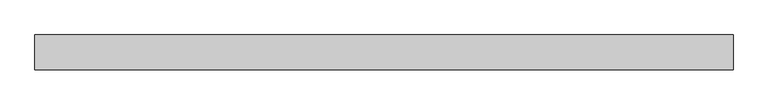
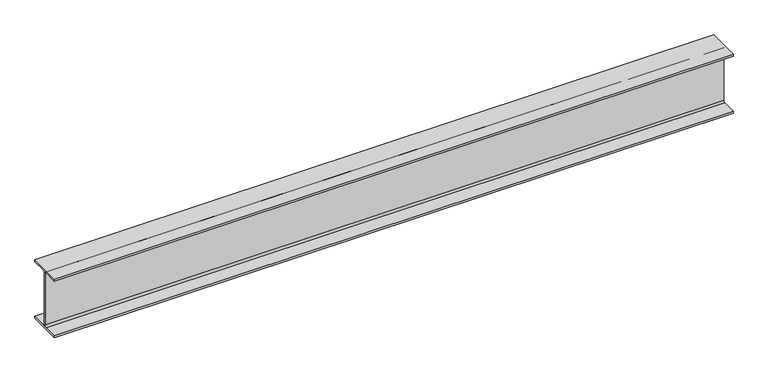
"""IFC4 building model written with IfcOpenShell, lengths in millimetres: beam geometry, Steel Beam_H-KSD3502 : H_SB_ASB_H-200x200x8x12."""

import ifcopenshell
import ifcopenshell.guid

model = None  # the IFC model being written
_history = None  # IfcOwnerHistory: only IFC2X3 demands one
_inside = {}  # id of a spatial element -> (the spatial element, [elements in it])
_under = {}  # id of a project, library or spatial element -> (it, [spatial elements below it])
_declared = {}  # id of a project -> (the project, [libraries it declares])
_typed = {}  # id of a type object -> (the type object, [elements of that type])
_made_of = {}  # id of a material, layer set ... -> (it, [elements and type objects made of it])


def new_model(schema):
    """Start an empty IFC model of exactly this schema.

    Asked for "IFC4X3", IfcOpenShell would pick the latest addendum, in which some entities
    have other attributes; the version numbers below select the first issue.
    IFC2X3 requires an IfcOwnerHistory on every rooted entity: one is made here for all.
    """
    global model, _history
    if schema == "IFC4X3":
        model = ifcopenshell.file(schema_version=(4, 3, 0, 0))
    else:
        model = ifcopenshell.file(schema=schema)
    _inside.clear()
    _under.clear()
    _declared.clear()
    _typed.clear()
    _made_of.clear()
    _history = None
    if model.schema == "IFC2X3":
        org = make("IfcOrganization", Name="unknown")
        user = make(
            "IfcPersonAndOrganization",
            ThePerson=make("IfcPerson", FamilyName="unknown"),
            TheOrganization=org,
        )
        app = make(
            "IfcApplication",
            ApplicationDeveloper=org,
            Version="unknown",
            ApplicationFullName="unknown",
            ApplicationIdentifier="unknown",
        )
        _history = make(
            "IfcOwnerHistory",
            OwningUser=user,
            OwningApplication=app,
            ChangeAction="ADDED",
            CreationDate=0,
        )
    return model


def make(cls, **values):
    """One entity of the class cls with the attributes given. An attribute that is None is left unset."""
    return model.create_entity(
        cls, **{name: value for name, value in values.items() if value is not None}
    )


def rooted(cls, **values):
    """An entity with a GlobalId (a new one), such as an element, a storey or a relation."""
    return make(cls, GlobalId=ifcopenshell.guid.new(), OwnerHistory=_history, **values)


def si_unit(unit_type, name, prefix=None):
    """IfcSIUnit, for example si_unit("LENGTHUNIT", "METRE", prefix="MILLI")."""
    return make("IfcSIUnit", UnitType=unit_type, Prefix=prefix, Name=name)


def assignment(units):
    """IfcUnitAssignment: the units of a project."""
    return None if units is None else make("IfcUnitAssignment", Units=units)


def point(xyz):
    """IfcCartesianPoint."""
    return None if xyz is None else make("IfcCartesianPoint", Coordinates=xyz)


def direction(xyz):
    """IfcDirection."""
    return None if xyz is None else make("IfcDirection", DirectionRatios=xyz)


def frame(location, z_axis=None, x_axis=None):
    """IfcAxis2Placement3D, a coordinate frame: its origin and axes. An axis left out is left unset."""
    return make(
        "IfcAxis2Placement3D",
        Location=point(location),
        Axis=direction(z_axis),
        RefDirection=direction(x_axis),
    )


def frame_2d(location, x_axis=None):
    """IfcAxis2Placement2D, a coordinate frame in the plane: its origin and x axis."""
    return make(
        "IfcAxis2Placement2D", Location=point(location), RefDirection=direction(x_axis)
    )


def origin():
    """The frame at (0, 0, 0) with its axes left unset."""
    return frame((0.0, 0.0, 0.0))


def place(relative_to, where):
    """IfcLocalPlacement: puts the frame where relative to a parent placement (None: the world)."""
    return make(
        "IfcLocalPlacement", PlacementRelTo=relative_to, RelativePlacement=where
    )


def context(
    kind, dimensions, precision=None, world=None, true_north=None, identifier=None
):
    """IfcGeometricRepresentationContext, for example the 3D "Model" context."""
    return make(
        "IfcGeometricRepresentationContext",
        ContextIdentifier=identifier,
        ContextType=kind,
        CoordinateSpaceDimension=dimensions,
        Precision=precision,
        WorldCoordinateSystem=world,
        TrueNorth=true_north,
    )


def project(units=None, contexts=None):
    """IfcProject with its units and contexts."""
    return rooted(
        "IfcProject",
        Name="project",
        RepresentationContexts=contexts,
        UnitsInContext=assignment(units),
    )


def spatial(cls, under=None, at=None, **own):
    """A site, building, storey or space (cls), placed at a placement, below another one or the project."""
    s = rooted(cls, ObjectPlacement=at, **own)
    if under is not None:
        _under.setdefault(under.id(), (under, []))[1].append(s)
    return s


def polyline(points):
    """IfcPolyline through the points."""
    return make("IfcPolyline", Points=[point(p) for p in points])


def circle_curve(where, radius):
    """IfcCircle in the frame where."""
    return make("IfcCircle", Position=where, Radius=radius)


def trimmed(basis, trim1, trim2, sense, master):
    """IfcTrimmedCurve: the piece of a basis curve between two trims."""
    return make(
        "IfcTrimmedCurve",
        BasisCurve=basis,
        Trim1=trim1,
        Trim2=trim2,
        SenseAgreement=sense,
        MasterRepresentation=master,
    )


def segment(curve, same_sense, transition):
    """IfcCompositeCurveSegment."""
    return make(
        "IfcCompositeCurveSegment",
        Transition=transition,
        SameSense=same_sense,
        ParentCurve=curve,
    )


def composite_curve(segments, self_intersect=None):
    """IfcCompositeCurve: segments joined end to end."""
    return make("IfcCompositeCurve", Segments=segments, SelfIntersect=self_intersect)


def outline(outer, holes=None, kind="AREA"):
    """IfcArbitraryClosedProfileDef: a profile drawn as a closed curve; with holes, ...WithVoids."""
    if holes is None:
        return make("IfcArbitraryClosedProfileDef", ProfileType=kind, OuterCurve=outer)
    return make(
        "IfcArbitraryProfileDefWithVoids",
        ProfileType=kind,
        OuterCurve=outer,
        InnerCurves=holes,
    )


def extrude(swept, where, along, depth):
    """IfcExtrudedAreaSolid: the profile swept, set in the frame where, extruded along a direction by depth."""
    return make(
        "IfcExtrudedAreaSolid",
        SweptArea=swept,
        Position=where,
        ExtrudedDirection=direction(along),
        Depth=depth,
    )


def shape(context_of_items, identifier, shape_type, items):
    """IfcShapeRepresentation: the items that make up one representation, for example the "Body"."""
    return make(
        "IfcShapeRepresentation",
        ContextOfItems=context_of_items,
        RepresentationIdentifier=identifier,
        RepresentationType=shape_type,
        Items=items,
    )


def source(mapping_origin, context_of_items, identifier, shape_type, items):
    """IfcRepresentationMap: a shape defined once, which mapped items show again and again."""
    return make(
        "IfcRepresentationMap",
        MappingOrigin=mapping_origin,
        MappedRepresentation=shape(context_of_items, identifier, shape_type, items),
    )


def transform(
    local_origin,
    x_axis=None,
    y_axis=None,
    z_axis=None,
    scale=None,
    scale2=None,
    scale3=None,
    uniform=True,
):
    """IfcCartesianTransformationOperator3D, or its non-uniform kind. x_axis, y_axis, z_axis: its Axis1, 2, 3."""
    if uniform:
        return make(
            "IfcCartesianTransformationOperator3D",
            Axis1=direction(x_axis),
            Axis2=direction(y_axis),
            LocalOrigin=point(local_origin),
            Scale=scale,
            Axis3=direction(z_axis),
        )
    return make(
        "IfcCartesianTransformationOperator3DnonUniform",
        Axis1=direction(x_axis),
        Axis2=direction(y_axis),
        LocalOrigin=point(local_origin),
        Scale=scale,
        Axis3=direction(z_axis),
        Scale2=scale2,
        Scale3=scale3,
    )


def mapped(mapping_source, mapping_target):
    """IfcMappedItem: shows the shape of a source again, moved by a transform."""
    return make(
        "IfcMappedItem", MappingSource=mapping_source, MappingTarget=mapping_target
    )


def made_of(thing, what):
    """Note that an element or type object is made of a material, layer set ...; save() writes the relation."""
    if what is not None:
        _made_of.setdefault(what.id(), (what, []))[1].append(thing)
    return thing


def element(
    cls,
    number,
    at=None,
    inside=None,
    cuts=None,
    type_object=None,
    material=None,
    context=None,
    identifier="Body",
    shape_type=None,
    held_by="IfcProductDefinitionShape",
    body=None,
    shapes=None,
    **own,
):
    """One element of the class cls, such as IfcWall. Its Tag is "e" and its number.

    at: its placement. inside: the storey or other place that contains it. cuts: it is an
    opening in that element (IfcRelVoidsElement). A single representation is given by context,
    identifier, shape_type and body (its items); several are given by shapes. held_by: the class
    of the entity that holds the representations. save() writes the other relations.
    """
    e = rooted(cls, Tag="e%d" % number, ObjectPlacement=at, **own)
    if body is not None:
        shapes = [shape(context, identifier, shape_type, body)]
    if shapes is not None:
        e.Representation = make(held_by, Representations=shapes)
    if inside is not None:
        _inside.setdefault(inside.id(), (inside, []))[1].append(e)
    if cuts is not None:
        rooted(
            "IfcRelVoidsElement", RelatingBuildingElement=cuts, RelatedOpeningElement=e
        )
    if type_object is not None:
        _typed.setdefault(type_object.id(), (type_object, []))[1].append(e)
    return made_of(e, material)


def aggregate(whole, parts):
    """IfcRelAggregates: a whole, such as a stair, and the parts it consists of."""
    return rooted("IfcRelAggregates", RelatingObject=whole, RelatedObjects=parts)


def save(model, path):
    """Write the relations noted so far, then the file.

    IfcRelAggregates (storeys below a building ...), IfcRelContainedInSpatialStructure (elements
    in a storey), IfcRelDefinesByType, IfcRelAssociatesMaterial and IfcRelDeclares: one each for
    every whole, place, type object, material and project.
    """
    for whole, parts in _under.values():
        aggregate(whole, parts)
    for where, things in _inside.values():
        rooted(
            "IfcRelContainedInSpatialStructure",
            RelatedElements=things,
            RelatingStructure=where,
        )
    for kind, things in _typed.values():
        rooted("IfcRelDefinesByType", RelatedObjects=things, RelatingType=kind)
    for what, things in _made_of.values():
        rooted("IfcRelAssociatesMaterial", RelatedObjects=things, RelatingMaterial=what)
    for by, libraries in _declared.values():
        rooted("IfcRelDeclares", RelatingContext=by, RelatedDefinitions=libraries)
    model.write(path)


def beam_87a33373(model_context):
    return source(origin(), model_context, "Body", "SweptSolid", [
        extrude(outline(composite_curve([segment(polyline([(82.5, -141.5), (82.5, -151.7), (-82.5, -151.7), (-82.5, -141.5), (-11.9, -141.5)]), True, "CONTINUOUS"), segment(trimmed(circle_curve(frame_2d((-11.9, -132.6)), 8.9), [point((-11.9, -141.5))], [point((-3.0, -132.6))], True, "CARTESIAN"), True, "CONTINUOUS"), segment(polyline([(-3.0, -132.6), (-3.0, 132.6)]), True, "CONTINUOUS"), segment(trimmed(circle_curve(frame_2d((-11.9, 132.6)), 8.9), [point((-3.0, 132.6))], [point((-11.9, 141.5))], True, "CARTESIAN"), True, "CONTINUOUS"), segment(polyline([(-11.9, 141.5), (-82.5, 141.5), (-82.5, 151.7), (82.5, 151.7), (82.5, 141.5), (11.9, 141.5)]), True, "CONTINUOUS"), segment(trimmed(circle_curve(frame_2d((11.9, 132.6)), 8.9), [point((11.9, 141.5))], [point((3.0, 132.6))], True, "CARTESIAN"), True, "CONTINUOUS"), segment(polyline([(3.0, 132.6), (3.0, -132.6)]), True, "CONTINUOUS"), segment(trimmed(circle_curve(frame_2d((11.9, -132.6)), 8.9), [point((3.0, -132.6))], [point((11.9, -141.5))], True, "CARTESIAN"), True, "CONTINUOUS"), segment(polyline([(11.9, -141.5), (82.5, -141.5)]), True, "CONTINUOUS")], self_intersect=False)), frame((-1611.7677924, 0.0, 0.0), z_axis=(1.0, 0.0, 0.0), x_axis=(0.0, 1.0, 0.0)), (0.0, 0.0, 1.0), 3310.7044425),
    ])


if __name__ == "__main__":
    model = new_model("IFC4")
    model_context = context("Model", 3, world=origin())
    ifc_project = project(units=[si_unit("LENGTHUNIT", "METRE", prefix="MILLI")], contexts=[model_context])
    site = spatial("IfcSite", under=ifc_project)
    building = spatial("IfcBuilding", under=site)
    placement = place(None, origin())
    beam_shape = beam_87a33373(model_context)
    element("IfcBeam", 1, ObjectType="Steel Beam_H-KSD3502 : H_SB_ASB_H-200x200x8x12", at=placement, inside=building, context=model_context, shape_type="MappedRepresentation", body=[
        mapped(beam_shape, transform((0.0, 0.0, 0.0), x_axis=(1.0, 0.0, 0.0), y_axis=(0.0, 1.0, 0.0), z_axis=(0.0, 0.0, 1.0))),
    ])
    save(model, "model.ifc")

# Revit data of these elements
# Type "Steel Beam_H-KSD3502 : H_SB_ASB_H-200x200x8x12"
#   Width = 20.0 cm
#   Web Thickness = 0.8 cm
#   Web Fillet = 1.3 cm
#   Warping Constant = 141376.0 cm⁶
#   Torsional Moment of Inertia = 26.2485 cm⁴
#   Torsional Modulus = 1.0 cm³
#   Section Area = 63.53 cm²
#   Plastic Modulus weak axis = 244.0 cm³
#   Plastic Modulus strong axis = 525.0 cm³
#   Perimeter = 1.16 m²/m
#   Nominal Weight = 49.90 kgf/m
#   Moment of Inertia weak axis = 1600.00 cm⁴
#   Moment of Inertia strong axis = 4720.00 cm⁴
#   Height = 20.0 cm
#   Flange Thickness = 1.2 cm
#   Elastic Modulus weak axis = 160.0 cm³
#   Elastic Modulus strong axis = 472.0 cm³
#   Centroid Vertical = 10.0 cm
#   Centroid Horizontal = 10.0 cm
#   Length [instance default] = 1.5240 m
#   Structural Material [instance default] = Steel, 45-345
#   Assembly Code = ""
# Element 1 (IfcBeam, "Steel Beam_H-KSD3502 : H_SB_ASB_H-200x200x8x12")
#   Structural Material = none
# Materials
#   "Steel, 45-345": class "Metal", colour RGB 189 187 185, transparency 0, Description = "Steel 345 MPa", Cost = 0
